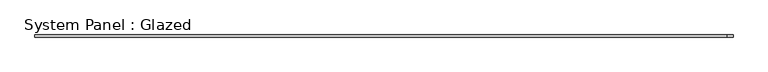
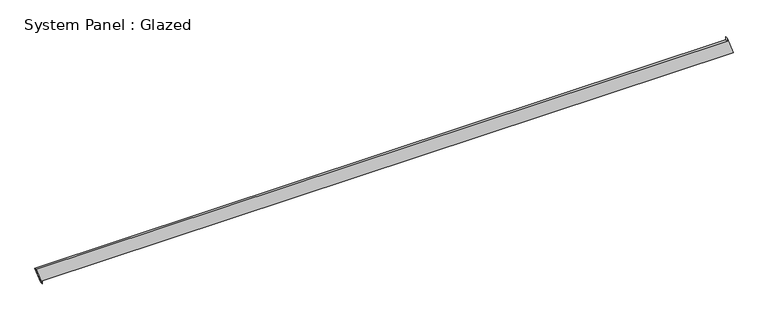
"""IFC4 building model written with IfcOpenShell, lengths in millimetres: plate geometry, System Panel : Glazed."""

from ifc_helpers import new_model, si_unit, frame, origin, place, context, project, spatial, polyline, outline, extrude, source, transform, mapped, element, save


def system_panel_glazed_b9c8f6ca(model_context):
    return source(origin(), model_context, "Body", "SweptSolid", [
        extrude(outline(polyline([(0.0, -3958.3006839), (35.3553391, -3958.3006839), (35.3553391, 4028.1117128), (235.2758426, 3958.2816454), (199.9205036, 3958.2816101), (199.9284866, -4028.1117128), (0.0, -3958.3006839)])), frame((0.0, -49.5, 0.0), z_axis=(0.0, 1.0, 0.0), x_axis=(0.0, 0.0, 1.0)), (0.0, 0.0, 1.0), 25.0),
    ])


if __name__ == "__main__":
    model = new_model("IFC4")
    model_context = context("Model", 3, world=origin())
    ifc_project = project(units=[si_unit("LENGTHUNIT", "METRE", prefix="MILLI")], contexts=[model_context])
    site = spatial("IfcSite", under=ifc_project)
    building = spatial("IfcBuilding", under=site)
    placement = place(None, origin())
    system_panel_glazed_shape = system_panel_glazed_b9c8f6ca(model_context)
    element("IfcPlate", 1, ObjectType="System Panel : Glazed", at=placement, inside=building, context=model_context, shape_type="MappedRepresentation", body=[
        mapped(system_panel_glazed_shape, transform((0.0, 0.0, 0.0), x_axis=(1.0, 0.0, 0.0), y_axis=(0.0, 1.0, 0.0), z_axis=(0.0, 0.0, 1.0))),
    ])
    save(model, "model.ifc")

# Revit data of these elements
# Element 1 (IfcPlate, "System Panel : Glazed")
#   Materials on its faces: "Glass"
# Materials
#   "Glass": class "Glass", colour RGB 218 227 224, transparency 0.85, Description = "Soda Lime Glass", Cost = 0
